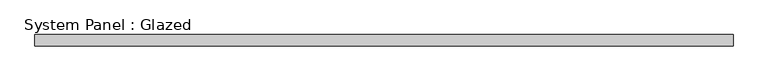
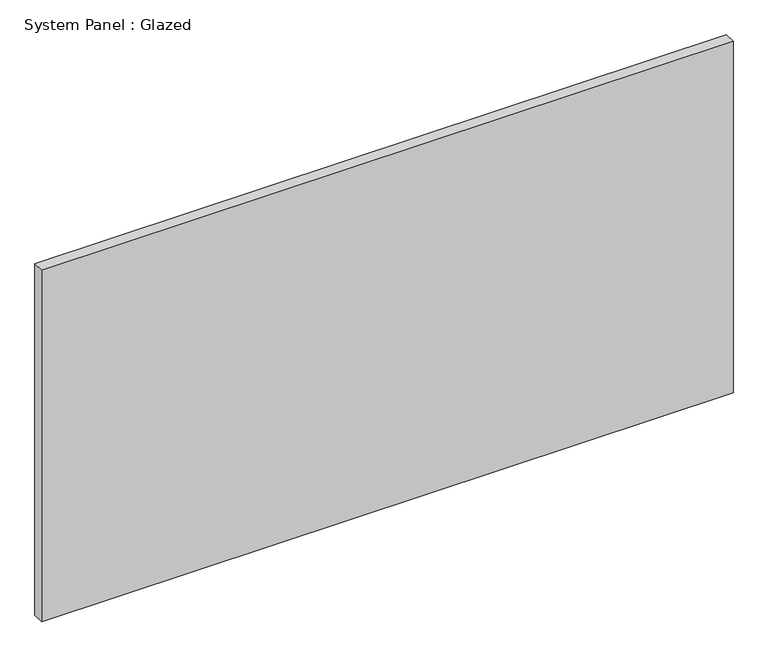
"""IFC4 building model written with IfcOpenShell, lengths in millimetres: plate geometry, System Panel : Glazed."""

from ifc_helpers import new_model, si_unit, origin, origin_with_axes, place, context, project, spatial, polyline, outline, extrude, source, transform, mapped, element, save


def system_panel_glazed_249c1314(model_context):
    return source(origin(), model_context, "Body", "SweptSolid", [
        extrude(outline(polyline([(768.3500002, -44.45), (-768.3500002, -44.45), (-768.3500002, -19.05), (768.3500002, -19.05), (768.3500002, -44.45)])), origin_with_axes(), (0.0, 0.0, 1.0), 825.5),
    ])


if __name__ == "__main__":
    model = new_model("IFC4")
    model_context = context("Model", 3, world=origin())
    ifc_project = project(units=[si_unit("LENGTHUNIT", "METRE", prefix="MILLI")], contexts=[model_context])
    site = spatial("IfcSite", under=ifc_project)
    building = spatial("IfcBuilding", under=site)
    placement = place(None, origin())
    system_panel_glazed_shape = system_panel_glazed_249c1314(model_context)
    element("IfcPlate", 1, ObjectType="System Panel : Glazed", at=placement, inside=building, context=model_context, shape_type="MappedRepresentation", body=[
        mapped(system_panel_glazed_shape, transform((0.0, 0.0, 0.0), x_axis=(1.0, 0.0, 0.0), y_axis=(0.0, 1.0, 0.0), z_axis=(0.0, 0.0, 1.0))),
    ])
    save(model, "model.ifc")

# Revit data of these elements
# Element 1 (IfcPlate, "System Panel : Glazed")
#   Materials on its faces: "Glass"
# Materials
#   "Glass": class "Glass", colour RGB 0 128 192, transparency 0.75
